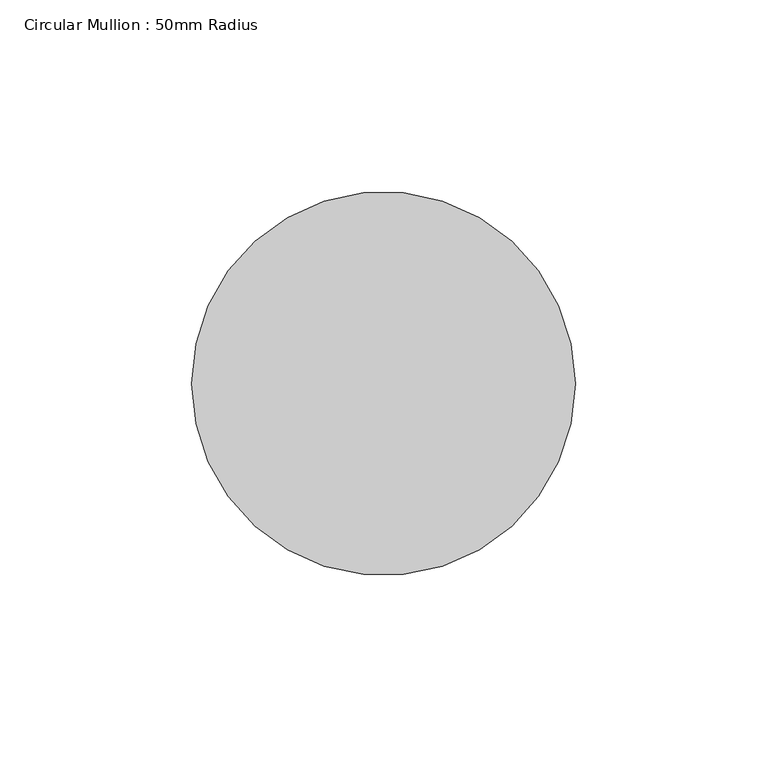
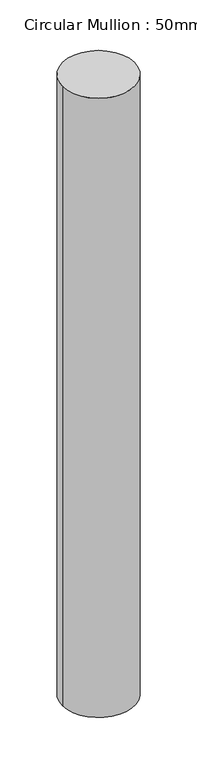
"""IFC4 building model written with IfcOpenShell, lengths in millimetres: member geometry, Circular Mullion : 50mm Radius."""

from ifc_helpers import new_model, si_unit, point, frame, origin, origin_2d, place, context, project, spatial, circle_curve, trimmed, segment, composite_curve, outline, extrude, source, transform, mapped, element, save


def circular_mullion_50mm_radius_625bf857(model_context):
    return source(origin(), model_context, "Body", "SweptSolid", [
        extrude(outline(composite_curve([segment(trimmed(circle_curve(origin_2d(), 50.0), [point((50.0, 0.0))], [point((-50.0, 0.0))], False, "CARTESIAN"), True, "CONTINUOUS"), segment(trimmed(circle_curve(origin_2d(), 50.0), [point((-50.0, 0.0))], [point((50.0, 0.0))], False, "CARTESIAN"), True, "CONTINUOUS")], self_intersect=False)), frame((0.0, 0.0, -905.8552067), z_axis=(0.0, 0.0, 1.0), x_axis=(1.0, 0.0, 0.0)), (0.0, 0.0, 1.0), 905.8552067),
    ])


if __name__ == "__main__":
    model = new_model("IFC4")
    model_context = context("Model", 3, world=origin())
    ifc_project = project(units=[si_unit("LENGTHUNIT", "METRE", prefix="MILLI")], contexts=[model_context])
    site = spatial("IfcSite", under=ifc_project)
    building = spatial("IfcBuilding", under=site)
    placement = place(None, origin())
    circular_mullion_50mm_radius_shape = circular_mullion_50mm_radius_625bf857(model_context)
    element("IfcMember", 1, ObjectType="Circular Mullion : 50mm Radius", at=placement, inside=building, context=model_context, shape_type="MappedRepresentation", body=[
        mapped(circular_mullion_50mm_radius_shape, transform((0.0, 0.0, 0.0), x_axis=(1.0, 0.0, 0.0), y_axis=(0.0, 1.0, 0.0), z_axis=(0.0, 0.0, 1.0))),
    ])
    save(model, "model.ifc")

# Revit data of these elements
# Type "Circular Mullion : 50mm Radius"
#   built-in parameter 1007350 = 0.164042 (stored number, unit not read)
# Element 1 (IfcMember, "Circular Mullion : 50mm Radius")
#   Materials on its faces: "Aluminium"
# Materials
#   "Aluminium": class "Metal", colour RGB 247 247 247, transparency 0, Description = "Aluminium 6061", Cost = 0
